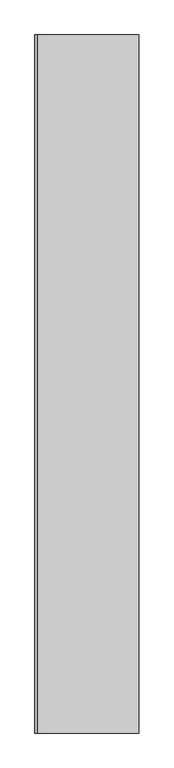
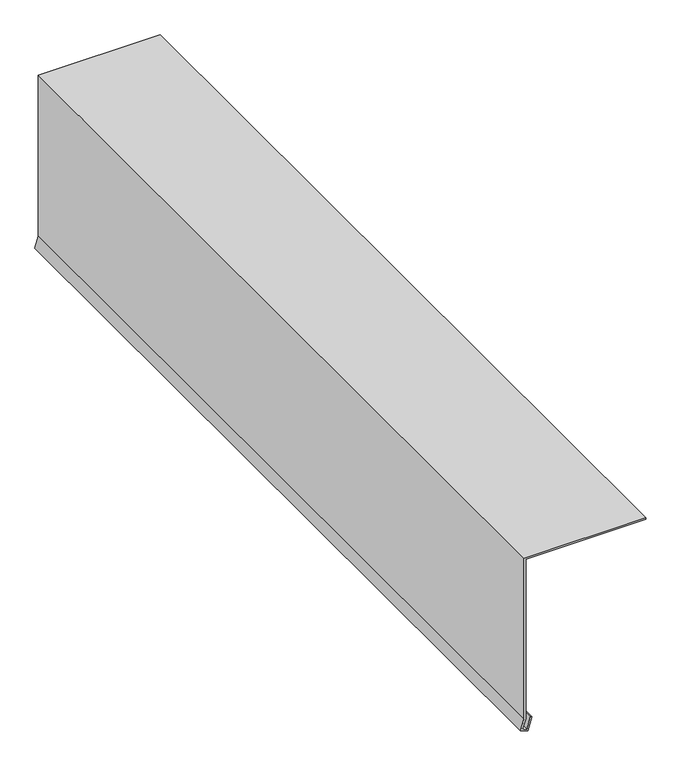
"""IFC4 building model written with IfcOpenShell, lengths in millimetres: proxy geometry, Flashing20:Flashing030:305752 : Flashing20:Flashing030:305752."""

from ifc_helpers import new_model, si_unit, frame, origin, place, context, project, spatial, polyline, outline, extrude, source, transform, mapped, element, save


def generic_models_cf6d0634(model_context):
    return source(origin(), model_context, "Body", "SweptSolid", [
        extrude(outline(polyline([(44157.1848954, 10085.7592949), (43752.7647284, 10085.7592949), (43725.7732624, 10077.4735459), (43720.3821423, 10095.0355351), (43751.7544661, 10104.7486666), (43752.9374956, 10100.9276142), (43725.3718611, 10092.3930653), (43728.4045857, 10082.4655275), (43752.1645952, 10089.7592949), (44153.1848954, 10089.7592949), (44153.1848954, 10375.5797727), (44157.1848954, 10375.5797727), (44157.1848954, 10085.7592949)])), frame((0.0, -774.5581163, 0.0), z_axis=(0.0, 1.0, 0.0), x_axis=(0.0, 0.0, 1.0)), (0.0, 0.0, 1.0), 1999.85),
    ])


if __name__ == "__main__":
    model = new_model("IFC4")
    model_context = context("Model", 3, world=origin())
    ifc_project = project(units=[si_unit("LENGTHUNIT", "METRE", prefix="MILLI")], contexts=[model_context])
    site = spatial("IfcSite", under=ifc_project)
    building = spatial("IfcBuilding", under=site)
    placement = place(None, origin())
    generic_models_shape = generic_models_cf6d0634(model_context)
    element("IfcBuildingElementProxy", 1, Name="Flashing20:Flashing030:305752 : Flashing20:Flashing030:305752", ObjectType="Flashing20:Flashing030:305752 : Flashing20:Flashing030:305752", at=placement, inside=building, context=model_context, shape_type="MappedRepresentation", body=[
        mapped(generic_models_shape, transform((0.0, 0.0, 0.0), x_axis=(1.0, 0.0, 0.0), y_axis=(0.0, 1.0, 0.0), z_axis=(0.0, 0.0, 1.0))),
    ])
    save(model, "model.ifc")

# Revit data of these elements
# Type "Flashing20:Flashing030:305752 : Flashing20:Flashing030:305752"
#   NameOverride = "Flashing20:Flashing030:305752"
#   ObjectTypeOverride = "Flashing20:Flashing030"
#   Reference = "Flashing030"
#   Category = "Generic Models"
#   Tag = "305752"
# Element 1 (IfcBuildingElementProxy, "Flashing20:Flashing030:305752 : Flashing20:Flashing030:305752")
#   Materials on its faces: "BRAKE METAL EAVE TRIM TO MATCH STANDING SEAM COLOR"
# Materials
#   "BRAKE METAL EAVE TRIM TO MATCH STANDING SEAM COLOR": class "Unassigned", colour RGB 128 128 128, transparency 0, Cost = 0
